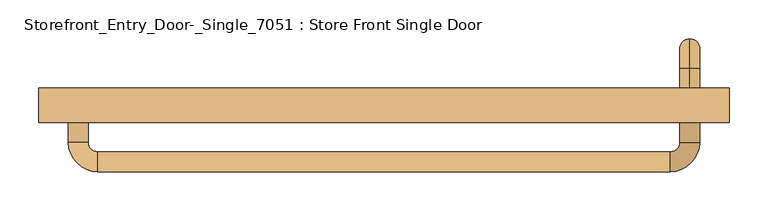
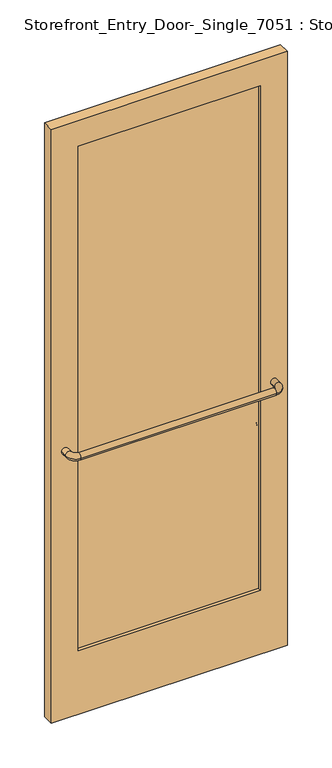
"""IFC4 building model written with IfcOpenShell, lengths in millimetres: door geometry, Storefront_Entry_Door-_Single_7051 : Store Front Single Door."""

import ifcopenshell
import ifcopenshell.guid

model = None  # the IFC model being written
_history = None  # IfcOwnerHistory: only IFC2X3 demands one
_inside = {}  # id of a spatial element -> (the spatial element, [elements in it])
_under = {}  # id of a project, library or spatial element -> (it, [spatial elements below it])
_declared = {}  # id of a project -> (the project, [libraries it declares])
_typed = {}  # id of a type object -> (the type object, [elements of that type])
_made_of = {}  # id of a material, layer set ... -> (it, [elements and type objects made of it])


def new_model(schema):
    """Start an empty IFC model of exactly this schema.

    Asked for "IFC4X3", IfcOpenShell would pick the latest addendum, in which some entities
    have other attributes; the version numbers below select the first issue.
    IFC2X3 requires an IfcOwnerHistory on every rooted entity: one is made here for all.
    """
    global model, _history
    if schema == "IFC4X3":
        model = ifcopenshell.file(schema_version=(4, 3, 0, 0))
    else:
        model = ifcopenshell.file(schema=schema)
    _inside.clear()
    _under.clear()
    _declared.clear()
    _typed.clear()
    _made_of.clear()
    _history = None
    if model.schema == "IFC2X3":
        org = make("IfcOrganization", Name="unknown")
        user = make(
            "IfcPersonAndOrganization",
            ThePerson=make("IfcPerson", FamilyName="unknown"),
            TheOrganization=org,
        )
        app = make(
            "IfcApplication",
            ApplicationDeveloper=org,
            Version="unknown",
            ApplicationFullName="unknown",
            ApplicationIdentifier="unknown",
        )
        _history = make(
            "IfcOwnerHistory",
            OwningUser=user,
            OwningApplication=app,
            ChangeAction="ADDED",
            CreationDate=0,
        )
    return model


def make(cls, **values):
    """One entity of the class cls with the attributes given. An attribute that is None is left unset."""
    return model.create_entity(
        cls, **{name: value for name, value in values.items() if value is not None}
    )


def rooted(cls, **values):
    """An entity with a GlobalId (a new one), such as an element, a storey or a relation."""
    return make(cls, GlobalId=ifcopenshell.guid.new(), OwnerHistory=_history, **values)


def si_unit(unit_type, name, prefix=None):
    """IfcSIUnit, for example si_unit("LENGTHUNIT", "METRE", prefix="MILLI")."""
    return make("IfcSIUnit", UnitType=unit_type, Prefix=prefix, Name=name)


def assignment(units):
    """IfcUnitAssignment: the units of a project."""
    return None if units is None else make("IfcUnitAssignment", Units=units)


def point(xyz):
    """IfcCartesianPoint."""
    return None if xyz is None else make("IfcCartesianPoint", Coordinates=xyz)


def direction(xyz):
    """IfcDirection."""
    return None if xyz is None else make("IfcDirection", DirectionRatios=xyz)


def frame(location, z_axis=None, x_axis=None):
    """IfcAxis2Placement3D, a coordinate frame: its origin and axes. An axis left out is left unset."""
    return make(
        "IfcAxis2Placement3D",
        Location=point(location),
        Axis=direction(z_axis),
        RefDirection=direction(x_axis),
    )


def origin():
    """The frame at (0, 0, 0) with its axes left unset."""
    return frame((0.0, 0.0, 0.0))


def place(relative_to, where):
    """IfcLocalPlacement: puts the frame where relative to a parent placement (None: the world)."""
    return make(
        "IfcLocalPlacement", PlacementRelTo=relative_to, RelativePlacement=where
    )


def context(
    kind, dimensions, precision=None, world=None, true_north=None, identifier=None
):
    """IfcGeometricRepresentationContext, for example the 3D "Model" context."""
    return make(
        "IfcGeometricRepresentationContext",
        ContextIdentifier=identifier,
        ContextType=kind,
        CoordinateSpaceDimension=dimensions,
        Precision=precision,
        WorldCoordinateSystem=world,
        TrueNorth=true_north,
    )


def project(units=None, contexts=None):
    """IfcProject with its units and contexts."""
    return rooted(
        "IfcProject",
        Name="project",
        RepresentationContexts=contexts,
        UnitsInContext=assignment(units),
    )


def spatial(cls, under=None, at=None, **own):
    """A site, building, storey or space (cls), placed at a placement, below another one or the project."""
    s = rooted(cls, ObjectPlacement=at, **own)
    if under is not None:
        _under.setdefault(under.id(), (under, []))[1].append(s)
    return s


def polyline(points):
    """IfcPolyline through the points."""
    return make("IfcPolyline", Points=[point(p) for p in points])


def circle_curve(where, radius):
    """IfcCircle in the frame where."""
    return make("IfcCircle", Position=where, Radius=radius)


def ellipse_curve(where, semi_axis1, semi_axis2):
    """IfcEllipse in the frame where."""
    return make(
        "IfcEllipse", Position=where, SemiAxis1=semi_axis1, SemiAxis2=semi_axis2
    )


def trimmed(basis, trim1, trim2, sense, master):
    """IfcTrimmedCurve: the piece of a basis curve between two trims."""
    return make(
        "IfcTrimmedCurve",
        BasisCurve=basis,
        Trim1=trim1,
        Trim2=trim2,
        SenseAgreement=sense,
        MasterRepresentation=master,
    )


def outline(outer, holes=None, kind="AREA"):
    """IfcArbitraryClosedProfileDef: a profile drawn as a closed curve; with holes, ...WithVoids."""
    if holes is None:
        return make("IfcArbitraryClosedProfileDef", ProfileType=kind, OuterCurve=outer)
    return make(
        "IfcArbitraryProfileDefWithVoids",
        ProfileType=kind,
        OuterCurve=outer,
        InnerCurves=holes,
    )


def extrude(swept, where, along, depth):
    """IfcExtrudedAreaSolid: the profile swept, set in the frame where, extruded along a direction by depth."""
    return make(
        "IfcExtrudedAreaSolid",
        SweptArea=swept,
        Position=where,
        ExtrudedDirection=direction(along),
        Depth=depth,
    )


def shape(context_of_items, identifier, shape_type, items):
    """IfcShapeRepresentation: the items that make up one representation, for example the "Body"."""
    return make(
        "IfcShapeRepresentation",
        ContextOfItems=context_of_items,
        RepresentationIdentifier=identifier,
        RepresentationType=shape_type,
        Items=items,
    )


def source(mapping_origin, context_of_items, identifier, shape_type, items):
    """IfcRepresentationMap: a shape defined once, which mapped items show again and again."""
    return make(
        "IfcRepresentationMap",
        MappingOrigin=mapping_origin,
        MappedRepresentation=shape(context_of_items, identifier, shape_type, items),
    )


def transform(
    local_origin,
    x_axis=None,
    y_axis=None,
    z_axis=None,
    scale=None,
    scale2=None,
    scale3=None,
    uniform=True,
):
    """IfcCartesianTransformationOperator3D, or its non-uniform kind. x_axis, y_axis, z_axis: its Axis1, 2, 3."""
    if uniform:
        return make(
            "IfcCartesianTransformationOperator3D",
            Axis1=direction(x_axis),
            Axis2=direction(y_axis),
            LocalOrigin=point(local_origin),
            Scale=scale,
            Axis3=direction(z_axis),
        )
    return make(
        "IfcCartesianTransformationOperator3DnonUniform",
        Axis1=direction(x_axis),
        Axis2=direction(y_axis),
        LocalOrigin=point(local_origin),
        Scale=scale,
        Axis3=direction(z_axis),
        Scale2=scale2,
        Scale3=scale3,
    )


def mapped(mapping_source, mapping_target):
    """IfcMappedItem: shows the shape of a source again, moved by a transform."""
    return make(
        "IfcMappedItem", MappingSource=mapping_source, MappingTarget=mapping_target
    )


def made_of(thing, what):
    """Note that an element or type object is made of a material, layer set ...; save() writes the relation."""
    if what is not None:
        _made_of.setdefault(what.id(), (what, []))[1].append(thing)
    return thing


def element(
    cls,
    number,
    at=None,
    inside=None,
    cuts=None,
    type_object=None,
    material=None,
    context=None,
    identifier="Body",
    shape_type=None,
    held_by="IfcProductDefinitionShape",
    body=None,
    shapes=None,
    **own,
):
    """One element of the class cls, such as IfcWall. Its Tag is "e" and its number.

    at: its placement. inside: the storey or other place that contains it. cuts: it is an
    opening in that element (IfcRelVoidsElement). A single representation is given by context,
    identifier, shape_type and body (its items); several are given by shapes. held_by: the class
    of the entity that holds the representations. save() writes the other relations.
    """
    e = rooted(cls, Tag="e%d" % number, ObjectPlacement=at, **own)
    if body is not None:
        shapes = [shape(context, identifier, shape_type, body)]
    if shapes is not None:
        e.Representation = make(held_by, Representations=shapes)
    if inside is not None:
        _inside.setdefault(inside.id(), (inside, []))[1].append(e)
    if cuts is not None:
        rooted(
            "IfcRelVoidsElement", RelatingBuildingElement=cuts, RelatedOpeningElement=e
        )
    if type_object is not None:
        _typed.setdefault(type_object.id(), (type_object, []))[1].append(e)
    return made_of(e, material)


def aggregate(whole, parts):
    """IfcRelAggregates: a whole, such as a stair, and the parts it consists of."""
    return rooted("IfcRelAggregates", RelatingObject=whole, RelatedObjects=parts)


def save(model, path):
    """Write the relations noted so far, then the file.

    IfcRelAggregates (storeys below a building ...), IfcRelContainedInSpatialStructure (elements
    in a storey), IfcRelDefinesByType, IfcRelAssociatesMaterial and IfcRelDeclares: one each for
    every whole, place, type object, material and project.
    """
    for whole, parts in _under.values():
        aggregate(whole, parts)
    for where, things in _inside.values():
        rooted(
            "IfcRelContainedInSpatialStructure",
            RelatedElements=things,
            RelatingStructure=where,
        )
    for kind, things in _typed.values():
        rooted("IfcRelDefinesByType", RelatedObjects=things, RelatingType=kind)
    for what, things in _made_of.values():
        rooted("IfcRelAssociatesMaterial", RelatedObjects=things, RelatingMaterial=what)
    for by, libraries in _declared.values():
        rooted("IfcRelDeclares", RelatingContext=by, RelatedDefinitions=libraries)
    model.write(path)


def plane_surface(at):
    """IfcPlane: the flat surface through the origin of the frame at, square to its z axis."""
    return make("IfcPlane", Position=at)


def cylinder_surface(at, radius):
    """IfcCylindricalSurface: all points at the distance radius from the z axis of the frame at."""
    return make("IfcCylindricalSurface", Position=at, Radius=radius)


def revolved_surface(curve, axis_point, axis_direction):
    """IfcSurfaceOfRevolution: the curve turned about the line through axis_point along axis_direction."""
    return make(
        "IfcSurfaceOfRevolution",
        SweptCurve=make("IfcArbitraryOpenProfileDef", ProfileType="CURVE", Curve=curve),
        AxisPosition=make("IfcAxis1Placement", Location=point(axis_point), Axis=direction(axis_direction)),
    )


def advanced_brep(points, edges, surfaces, faces):
    """IfcAdvancedBrep: a solid bounded by faces that lie on surfaces and meet in shared edges.

    An edge is (start, end): straight between two places in points (the first is 0);
    or (start, end, curve); or (start, end, curve, False) where it runs against its curve.
    A face is (place in surfaces, loops), or (place, loops, False) where it looks against
    its surface's normal. A loop lists edges by number (the first is 1), with a minus sign
    where the edge is run from its end to its start. The first loop is the outer one.
    """
    corners = [point(p) for p in points]
    vertices = [make("IfcVertexPoint", VertexGeometry=c) for c in corners]
    made = []
    for start, end, *more in edges:
        made.append(
            make(
                "IfcEdgeCurve",
                EdgeStart=vertices[start],
                EdgeEnd=vertices[end],
                EdgeGeometry=more[0] if more else make("IfcPolyline", Points=[corners[start], corners[end]]),
                SameSense=more[1] if len(more) > 1 else True,
            )
        )
    hull = []
    for where, loops, *sense in faces:
        bounds = []
        for j, loop in enumerate(loops):
            ring = [make("IfcOrientedEdge", EdgeElement=made[abs(k) - 1], Orientation=k > 0) for k in loop]
            bounds.append(
                make(
                    "IfcFaceOuterBound" if j == 0 else "IfcFaceBound",
                    Bound=make("IfcEdgeLoop", EdgeList=ring),
                    Orientation=True,
                )
            )
        hull.append(make("IfcAdvancedFace", Bounds=bounds, FaceSurface=surfaces[where], SameSense=sense[0] if sense else True))
    return make("IfcAdvancedBrep", Outer=make("IfcClosedShell", CfsFaces=hull))


def storefront_entry_door_single_7051_store_front_single_door_8ffc33a8(model_context):
    return source(origin(), model_context, "Body", "SolidModel", [
        advanced_brep(
        [(393.7, 50.8, 1054.1), (393.7, 50.8, 1079.5), (393.7, 76.2, 1054.1), (393.7, 76.2, 1079.5), (393.7, 114.3, 1041.4), (393.7, 88.9, 1041.4), (393.7, 88.9, 863.6), (393.7, 114.3, 863.6), (393.7, 76.2, 825.5), (393.7, 76.2, 850.9), (393.7, 50.8, 850.9), (393.7, 50.8, 825.5)],
        [
            (0, 1, circle_curve(frame((393.7, 50.8, 1066.8), z_axis=(0.0, -1.0, 0.0), x_axis=(0.0, 0.0, 1.0)), 12.7)),
            (1, 0, circle_curve(frame((393.7, 50.8, 1066.8), z_axis=(0.0, -1.0, 0.0), x_axis=(0.0, 0.0, 1.0)), 12.7)),
            (0, 2),
            (2, 3, circle_curve(frame((393.7, 76.2, 1066.8), z_axis=(0.0, -1.0, 0.0), x_axis=(0.0, 0.0, 1.0)), 12.7)),
            (3, 1),
            (3, 2, circle_curve(frame((393.7, 76.2, 1066.8), z_axis=(0.0, -1.0, 0.0), x_axis=(0.0, 0.0, 1.0)), 12.7)),
            (4, 3, circle_curve(frame((393.7, 76.2, 1041.4), z_axis=(1.0, 0.0, 0.0), x_axis=(0.0, 0.0, 1.0)), 38.1)),
            (2, 5, circle_curve(frame((393.7, 76.2, 1041.4), z_axis=(-1.0, 0.0, 0.0), x_axis=(0.0, 0.0, 1.0)), 12.7)),
            (5, 4, circle_curve(frame((393.7, 101.6, 1041.4), z_axis=(0.0, 0.0, 1.0), x_axis=(0.0, 1.0, 0.0)), 12.7)),
            (4, 5, circle_curve(frame((393.7, 101.6, 1041.4), z_axis=(0.0, 0.0, 1.0), x_axis=(0.0, 1.0, 0.0)), 12.7)),
            (5, 6),
            (6, 7, circle_curve(frame((393.7, 101.6, 863.6), z_axis=(0.0, 0.0, 1.0), x_axis=(0.0, 1.0, 0.0)), 12.7)),
            (7, 4),
            (7, 6, circle_curve(frame((393.7, 101.6, 863.6), z_axis=(0.0, 0.0, 1.0), x_axis=(0.0, 1.0, 0.0)), 12.7)),
            (8, 7, circle_curve(frame((393.7, 76.2, 863.6), z_axis=(1.0, 0.0, 0.0), x_axis=(0.0, 1.0, 0.0)), 38.1)),
            (6, 9, circle_curve(frame((393.7, 76.2, 863.6), z_axis=(-1.0, 0.0, 0.0), x_axis=(0.0, 1.0, 0.0)), 12.7)),
            (9, 8, circle_curve(frame((393.7, 76.2, 838.2), z_axis=(0.0, 1.0, 0.0), x_axis=(0.0, 0.0, -1.0)), 12.7)),
            (8, 9, circle_curve(frame((393.7, 76.2, 838.2), z_axis=(0.0, 1.0, 0.0), x_axis=(0.0, 0.0, -1.0)), 12.7)),
            (10, 11, circle_curve(frame((393.7, 50.8, 838.2), z_axis=(0.0, -1.0, 0.0), x_axis=(0.0, 0.0, -1.0)), 12.7)),
            (11, 10, circle_curve(frame((393.7, 50.8, 838.2), z_axis=(0.0, -1.0, 0.0), x_axis=(0.0, 0.0, -1.0)), 12.7)),
            (9, 10),
            (11, 8),
        ],
        [
            plane_surface(frame((393.7, 50.8, 1066.8), z_axis=(0.0, -1.0, 0.0), x_axis=(1.0, 0.0, 0.0))),
            cylinder_surface(frame((393.7, 50.8, 1066.8), z_axis=(0.0, -1.0, 0.0), x_axis=(0.0, 0.0, 1.0)), 12.7),
            revolved_surface(trimmed(ellipse_curve(frame((393.7, 76.2, 1066.8), z_axis=(0.0, -1.0, 0.0), x_axis=(0.0, 0.0, 1.0)), 12.7, 12.7), [point((393.7, 76.2, 1054.1))], [point((393.7, 76.2, 1079.5))], True, "CARTESIAN"), (393.7, 76.2, 1041.4), (-1.0, 0.0, 0.0)),
            revolved_surface(trimmed(ellipse_curve(frame((393.7, 76.2, 1066.8), z_axis=(0.0, -1.0, 0.0), x_axis=(0.0, 0.0, 1.0)), 12.7, 12.7), [point((393.7, 76.2, 1079.5))], [point((393.7, 76.2, 1054.1))], True, "CARTESIAN"), (393.7, 76.2, 1041.4), (-1.0, 0.0, 0.0)),
            cylinder_surface(frame((393.7, 101.6, 1041.4), z_axis=(0.0, 0.0, 1.0), x_axis=(0.0, 1.0, 0.0)), 12.7),
            revolved_surface(trimmed(ellipse_curve(frame((393.7, 101.6, 863.6), z_axis=(0.0, 0.0, 1.0), x_axis=(0.0, 1.0, 0.0)), 12.7, 12.7), [point((393.7, 88.9, 863.6))], [point((393.7, 114.3, 863.6))], True, "CARTESIAN"), (393.7, 76.2, 863.6), (-1.0, 0.0, 0.0)),
            revolved_surface(trimmed(ellipse_curve(frame((393.7, 101.6, 863.6), z_axis=(0.0, 0.0, 1.0), x_axis=(0.0, 1.0, 0.0)), 12.7, 12.7), [point((393.7, 114.3, 863.6))], [point((393.7, 88.9, 863.6))], True, "CARTESIAN"), (393.7, 76.2, 863.6), (-1.0, 0.0, 0.0)),
            plane_surface(frame((393.7, 50.8, 838.2), z_axis=(0.0, -1.0, 0.0), x_axis=(1.0, 0.0, 0.0))),
            cylinder_surface(frame((393.7, 76.2, 838.2), z_axis=(0.0, 1.0, 0.0), x_axis=(0.0, 0.0, -1.0)), 12.7),
        ],
        [
            (0, [[1, 2]]),
            (1, [[-1, 3, 4, 5]]),
            (1, [[-2, -5, 6, -3]]),
            (2, [[7, -4, 8, 9]]),
            (3, [[-8, -6, -7, 10]]),
            (4, [[-9, 11, 12, 13]]),
            (4, [[-10, -13, 14, -11]]),
            (5, [[15, -12, 16, 17]]),
            (6, [[-16, -14, -15, 18]]),
            (7, [[19, 20]]),
            (8, [[-17, 21, -20, 22]]),
            (8, [[-18, -22, -19, -21]]),
        ],
    ),
        advanced_brep(
        [(381.0, 6.35, 1066.8), (406.4, 6.35, 1066.8), (381.0, -19.05, 1066.8), (406.4, -19.05, 1066.8), (368.3, -57.15, 1066.8), (368.3, -31.75, 1066.8), (-368.3, -31.75, 1066.8), (-368.3, -57.15, 1066.8), (-406.4, -19.05, 1066.8), (-381.0, -19.05, 1066.8), (-381.0, 6.35, 1066.8), (-406.4, 6.35, 1066.8)],
        [
            (0, 1, circle_curve(frame((393.7, 6.35, 1066.8), z_axis=(0.0, 1.0, 0.0), x_axis=(1.0, 0.0, 0.0)), 12.7)),
            (1, 0, circle_curve(frame((393.7, 6.35, 1066.8), z_axis=(0.0, 1.0, 0.0), x_axis=(1.0, 0.0, 0.0)), 12.7)),
            (0, 2),
            (2, 3, circle_curve(frame((393.7, -19.05, 1066.8), z_axis=(0.0, 1.0, 0.0), x_axis=(1.0, 0.0, 0.0)), 12.7)),
            (3, 1),
            (3, 2, circle_curve(frame((393.7, -19.05, 1066.8), z_axis=(0.0, 1.0, 0.0), x_axis=(1.0, 0.0, 0.0)), 12.7)),
            (4, 3, circle_curve(frame((368.3, -19.05, 1066.8), z_axis=(0.0, 0.0, 1.0), x_axis=(1.0, 0.0, 0.0)), 38.1)),
            (2, 5, circle_curve(frame((368.3, -19.05, 1066.8), z_axis=(0.0, 0.0, -1.0), x_axis=(1.0, 0.0, 0.0)), 12.7)),
            (5, 4, circle_curve(frame((368.3, -44.45, 1066.8), z_axis=(1.0, 0.0, 0.0), x_axis=(0.0, -1.0, 0.0)), 12.7)),
            (4, 5, circle_curve(frame((368.3, -44.45, 1066.8), z_axis=(1.0, 0.0, 0.0), x_axis=(0.0, -1.0, 0.0)), 12.7)),
            (5, 6),
            (6, 7, circle_curve(frame((-368.3, -44.45, 1066.8), z_axis=(1.0, 0.0, 0.0), x_axis=(0.0, -1.0, 0.0)), 12.7)),
            (7, 4),
            (7, 6, circle_curve(frame((-368.3, -44.45, 1066.8), z_axis=(1.0, 0.0, 0.0), x_axis=(0.0, -1.0, 0.0)), 12.7)),
            (8, 7, circle_curve(frame((-368.3, -19.05, 1066.8), z_axis=(0.0, 0.0, 1.0), x_axis=(0.0, -1.0, 0.0)), 38.1)),
            (6, 9, circle_curve(frame((-368.3, -19.05, 1066.8), z_axis=(0.0, 0.0, -1.0), x_axis=(0.0, -1.0, 0.0)), 12.7)),
            (9, 8, circle_curve(frame((-393.7, -19.05, 1066.8), z_axis=(0.0, -1.0, 0.0), x_axis=(-1.0, 0.0, 0.0)), 12.7)),
            (8, 9, circle_curve(frame((-393.7, -19.05, 1066.8), z_axis=(0.0, -1.0, 0.0), x_axis=(-1.0, 0.0, 0.0)), 12.7)),
            (10, 11, circle_curve(frame((-393.7, 6.35, 1066.8), z_axis=(0.0, 1.0, 0.0), x_axis=(-1.0, 0.0, 0.0)), 12.7)),
            (11, 10, circle_curve(frame((-393.7, 6.35, 1066.8), z_axis=(0.0, 1.0, 0.0), x_axis=(-1.0, 0.0, 0.0)), 12.7)),
            (9, 10),
            (11, 8),
        ],
        [
            plane_surface(frame((393.7, 6.35, 1066.8), z_axis=(0.0, 1.0, 0.0), x_axis=(0.0, 0.0, 1.0))),
            cylinder_surface(frame((393.7, 6.35, 1066.8), z_axis=(0.0, 1.0, 0.0), x_axis=(1.0, 0.0, 0.0)), 12.7),
            revolved_surface(trimmed(ellipse_curve(frame((393.7, -19.05, 1066.8), z_axis=(0.0, 1.0, 0.0), x_axis=(1.0, 0.0, 0.0)), 12.7, 12.7), [point((381.0, -19.05, 1066.8))], [point((406.4, -19.05, 1066.8))], True, "CARTESIAN"), (368.3, -19.05, 1066.8), (0.0, 0.0, -1.0)),
            revolved_surface(trimmed(ellipse_curve(frame((393.7, -19.05, 1066.8), z_axis=(0.0, 1.0, 0.0), x_axis=(1.0, 0.0, 0.0)), 12.7, 12.7), [point((406.4, -19.05, 1066.8))], [point((381.0, -19.05, 1066.8))], True, "CARTESIAN"), (368.3, -19.05, 1066.8), (0.0, 0.0, -1.0)),
            cylinder_surface(frame((368.3, -44.45, 1066.8), z_axis=(1.0, 0.0, 0.0), x_axis=(0.0, -1.0, 0.0)), 12.7),
            revolved_surface(trimmed(ellipse_curve(frame((-368.3, -44.45, 1066.8), z_axis=(1.0, 0.0, 0.0), x_axis=(0.0, -1.0, 0.0)), 12.7, 12.7), [point((-368.3, -31.75, 1066.8))], [point((-368.3, -57.15, 1066.8))], True, "CARTESIAN"), (-368.3, -19.05, 1066.8), (0.0, 0.0, -1.0)),
            revolved_surface(trimmed(ellipse_curve(frame((-368.3, -44.45, 1066.8), z_axis=(1.0, 0.0, 0.0), x_axis=(0.0, -1.0, 0.0)), 12.7, 12.7), [point((-368.3, -57.15, 1066.8))], [point((-368.3, -31.75, 1066.8))], True, "CARTESIAN"), (-368.3, -19.05, 1066.8), (0.0, 0.0, -1.0)),
            plane_surface(frame((-393.7, 6.35, 1066.8), z_axis=(0.0, 1.0, 0.0), x_axis=(0.0, 0.0, 1.0))),
            cylinder_surface(frame((-393.7, -19.05, 1066.8), z_axis=(0.0, -1.0, 0.0), x_axis=(-1.0, 0.0, 0.0)), 12.7),
        ],
        [
            (0, [[1, 2]]),
            (1, [[-1, 3, 4, 5]]),
            (1, [[-2, -5, 6, -3]]),
            (2, [[7, -4, 8, 9]]),
            (3, [[-8, -6, -7, 10]]),
            (4, [[-9, 11, 12, 13]]),
            (4, [[-10, -13, 14, -11]]),
            (5, [[15, -12, 16, 17]]),
            (6, [[-16, -14, -15, 18]]),
            (7, [[19, 20]]),
            (8, [[-17, 21, -20, 22]]),
            (8, [[-18, -22, -19, -21]]),
        ],
    ),
        extrude(outline(polyline([(342.9, 19.05), (-342.9, 19.05), (-342.9, 38.1), (342.9, 38.1), (342.9, 19.05)])), frame((0.0, 0.0, 254.0), z_axis=(0.0, 0.0, 1.0), x_axis=(1.0, 0.0, 0.0)), (0.0, 0.0, 1.0), 2006.6),
        extrude(outline(polyline([(2362.2, 444.5), (2362.2, -444.5), (0.0, -444.5), (0.0, 444.5), (2362.2, 444.5)]), holes=[polyline([(2260.6, -342.9), (2260.6, 342.9), (254.0, 342.9), (254.0, -342.9), (2260.6, -342.9)])]), frame((0.0, 6.35, 0.0), z_axis=(0.0, 1.0, 0.0), x_axis=(0.0, 0.0, 1.0)), (0.0, 0.0, 1.0), 44.45),
    ])


if __name__ == "__main__":
    model = new_model("IFC4")
    model_context = context("Model", 3, world=origin())
    ifc_project = project(units=[si_unit("LENGTHUNIT", "METRE", prefix="MILLI")], contexts=[model_context])
    site = spatial("IfcSite", under=ifc_project)
    building = spatial("IfcBuilding", under=site)
    placement = place(None, origin())
    storefront_entry_door_single_7051_store_front_single_door_shape = storefront_entry_door_single_7051_store_front_single_door_8ffc33a8(model_context)
    element("IfcDoor", 1, ObjectType="Storefront_Entry_Door-_Single_7051 : Store Front Single Door", at=placement, inside=building, context=model_context, shape_type="MappedRepresentation", body=[
        mapped(storefront_entry_door_single_7051_store_front_single_door_shape, transform((0.0, 0.0, 0.0), x_axis=(1.0, 0.0, 0.0), y_axis=(0.0, 1.0, 0.0), z_axis=(0.0, 0.0, 1.0))),
    ])
    save(model, "model.ifc")

# Revit data of these elements
# Type "Storefront_Entry_Door-_Single_7051 : Store Front Single Door"
#   Type Comments = "TEMPERED GLAZING"
#   Type Mark = "19"
#   Assembly Code = "B2030110"
#   Analytic Construction = "<None>"
#   Top Rail = 0' - 4"
#   Side Rail = 0' - 4"
#   Reporting Width [instance default] = 4' - 2"
#   Rail Height AFF = 3' - 6"
#   Offset = 0' - 2"
#   Door Width [instance default] = 4' - 2"
#   Bottom Rail Width = 0' - 10"
#   Material = Metal - Aluminum
#   Glazing Material = Glass
#   Function = (empty or 0)
# Element 1 (IfcDoor, "Storefront_Entry_Door-_Single_7051 : Store Front Single Door")
#   Reporting Width = 2' - 11"
#   Door Width = 2' - 11"
#   Materials on its faces: "Metal - Aluminum", "Glass"
# Materials
#   "Metal - Aluminum": class "Metal", colour RGB 247 247 247, transparency 0
#   "Glass": class "Glass", colour RGB 218 227 224, transparency 0.85, Description = "Soda Lime Glass", Cost = 0
